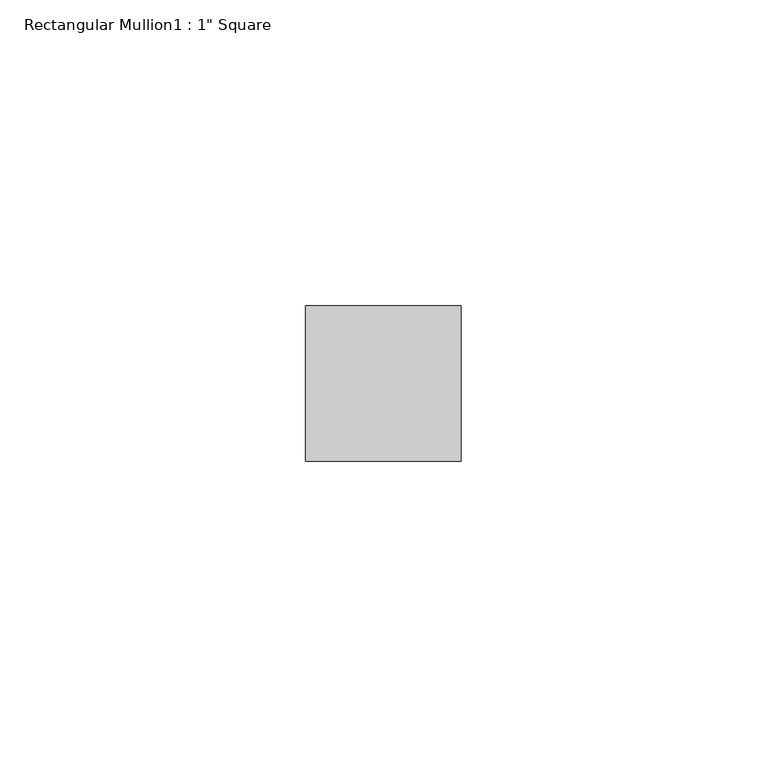
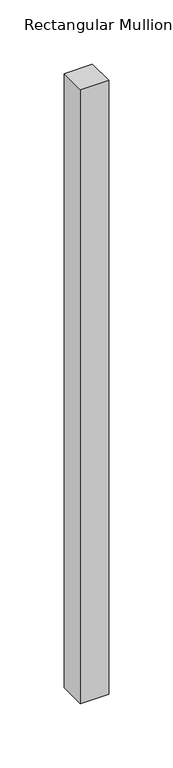
"""IFC4 building model written with IfcOpenShell, lengths in millimetres: member geometry."""

import ifcopenshell
import ifcopenshell.guid

model = None  # the IFC model being written
_history = None  # IfcOwnerHistory: only IFC2X3 demands one
_inside = {}  # id of a spatial element -> (the spatial element, [elements in it])
_under = {}  # id of a project, library or spatial element -> (it, [spatial elements below it])
_declared = {}  # id of a project -> (the project, [libraries it declares])
_typed = {}  # id of a type object -> (the type object, [elements of that type])
_made_of = {}  # id of a material, layer set ... -> (it, [elements and type objects made of it])


def new_model(schema):
    """Start an empty IFC model of exactly this schema.

    Asked for "IFC4X3", IfcOpenShell would pick the latest addendum, in which some entities
    have other attributes; the version numbers below select the first issue.
    IFC2X3 requires an IfcOwnerHistory on every rooted entity: one is made here for all.
    """
    global model, _history
    if schema == "IFC4X3":
        model = ifcopenshell.file(schema_version=(4, 3, 0, 0))
    else:
        model = ifcopenshell.file(schema=schema)
    _inside.clear()
    _under.clear()
    _declared.clear()
    _typed.clear()
    _made_of.clear()
    _history = None
    if model.schema == "IFC2X3":
        org = make("IfcOrganization", Name="unknown")
        user = make(
            "IfcPersonAndOrganization",
            ThePerson=make("IfcPerson", FamilyName="unknown"),
            TheOrganization=org,
        )
        app = make(
            "IfcApplication",
            ApplicationDeveloper=org,
            Version="unknown",
            ApplicationFullName="unknown",
            ApplicationIdentifier="unknown",
        )
        _history = make(
            "IfcOwnerHistory",
            OwningUser=user,
            OwningApplication=app,
            ChangeAction="ADDED",
            CreationDate=0,
        )
    return model


def make(cls, **values):
    """One entity of the class cls with the attributes given. An attribute that is None is left unset."""
    return model.create_entity(
        cls, **{name: value for name, value in values.items() if value is not None}
    )


def rooted(cls, **values):
    """An entity with a GlobalId (a new one), such as an element, a storey or a relation."""
    return make(cls, GlobalId=ifcopenshell.guid.new(), OwnerHistory=_history, **values)


def si_unit(unit_type, name, prefix=None):
    """IfcSIUnit, for example si_unit("LENGTHUNIT", "METRE", prefix="MILLI")."""
    return make("IfcSIUnit", UnitType=unit_type, Prefix=prefix, Name=name)


def assignment(units):
    """IfcUnitAssignment: the units of a project."""
    return None if units is None else make("IfcUnitAssignment", Units=units)


def point(xyz):
    """IfcCartesianPoint."""
    return None if xyz is None else make("IfcCartesianPoint", Coordinates=xyz)


def direction(xyz):
    """IfcDirection."""
    return None if xyz is None else make("IfcDirection", DirectionRatios=xyz)


def frame(location, z_axis=None, x_axis=None):
    """IfcAxis2Placement3D, a coordinate frame: its origin and axes. An axis left out is left unset."""
    return make(
        "IfcAxis2Placement3D",
        Location=point(location),
        Axis=direction(z_axis),
        RefDirection=direction(x_axis),
    )


def origin():
    """The frame at (0, 0, 0) with its axes left unset."""
    return frame((0.0, 0.0, 0.0))


def place(relative_to, where):
    """IfcLocalPlacement: puts the frame where relative to a parent placement (None: the world)."""
    return make(
        "IfcLocalPlacement", PlacementRelTo=relative_to, RelativePlacement=where
    )


def context(
    kind, dimensions, precision=None, world=None, true_north=None, identifier=None
):
    """IfcGeometricRepresentationContext, for example the 3D "Model" context."""
    return make(
        "IfcGeometricRepresentationContext",
        ContextIdentifier=identifier,
        ContextType=kind,
        CoordinateSpaceDimension=dimensions,
        Precision=precision,
        WorldCoordinateSystem=world,
        TrueNorth=true_north,
    )


def project(units=None, contexts=None):
    """IfcProject with its units and contexts."""
    return rooted(
        "IfcProject",
        Name="project",
        RepresentationContexts=contexts,
        UnitsInContext=assignment(units),
    )


def spatial(cls, under=None, at=None, **own):
    """A site, building, storey or space (cls), placed at a placement, below another one or the project."""
    s = rooted(cls, ObjectPlacement=at, **own)
    if under is not None:
        _under.setdefault(under.id(), (under, []))[1].append(s)
    return s


def polyline(points):
    """IfcPolyline through the points."""
    return make("IfcPolyline", Points=[point(p) for p in points])


def outline(outer, holes=None, kind="AREA"):
    """IfcArbitraryClosedProfileDef: a profile drawn as a closed curve; with holes, ...WithVoids."""
    if holes is None:
        return make("IfcArbitraryClosedProfileDef", ProfileType=kind, OuterCurve=outer)
    return make(
        "IfcArbitraryProfileDefWithVoids",
        ProfileType=kind,
        OuterCurve=outer,
        InnerCurves=holes,
    )


def extrude(swept, where, along, depth):
    """IfcExtrudedAreaSolid: the profile swept, set in the frame where, extruded along a direction by depth."""
    return make(
        "IfcExtrudedAreaSolid",
        SweptArea=swept,
        Position=where,
        ExtrudedDirection=direction(along),
        Depth=depth,
    )


def shape(context_of_items, identifier, shape_type, items):
    """IfcShapeRepresentation: the items that make up one representation, for example the "Body"."""
    return make(
        "IfcShapeRepresentation",
        ContextOfItems=context_of_items,
        RepresentationIdentifier=identifier,
        RepresentationType=shape_type,
        Items=items,
    )


def source(mapping_origin, context_of_items, identifier, shape_type, items):
    """IfcRepresentationMap: a shape defined once, which mapped items show again and again."""
    return make(
        "IfcRepresentationMap",
        MappingOrigin=mapping_origin,
        MappedRepresentation=shape(context_of_items, identifier, shape_type, items),
    )


def transform(
    local_origin,
    x_axis=None,
    y_axis=None,
    z_axis=None,
    scale=None,
    scale2=None,
    scale3=None,
    uniform=True,
):
    """IfcCartesianTransformationOperator3D, or its non-uniform kind. x_axis, y_axis, z_axis: its Axis1, 2, 3."""
    if uniform:
        return make(
            "IfcCartesianTransformationOperator3D",
            Axis1=direction(x_axis),
            Axis2=direction(y_axis),
            LocalOrigin=point(local_origin),
            Scale=scale,
            Axis3=direction(z_axis),
        )
    return make(
        "IfcCartesianTransformationOperator3DnonUniform",
        Axis1=direction(x_axis),
        Axis2=direction(y_axis),
        LocalOrigin=point(local_origin),
        Scale=scale,
        Axis3=direction(z_axis),
        Scale2=scale2,
        Scale3=scale3,
    )


def mapped(mapping_source, mapping_target):
    """IfcMappedItem: shows the shape of a source again, moved by a transform."""
    return make(
        "IfcMappedItem", MappingSource=mapping_source, MappingTarget=mapping_target
    )


def made_of(thing, what):
    """Note that an element or type object is made of a material, layer set ...; save() writes the relation."""
    if what is not None:
        _made_of.setdefault(what.id(), (what, []))[1].append(thing)
    return thing


def element(
    cls,
    number,
    at=None,
    inside=None,
    cuts=None,
    type_object=None,
    material=None,
    context=None,
    identifier="Body",
    shape_type=None,
    held_by="IfcProductDefinitionShape",
    body=None,
    shapes=None,
    **own,
):
    """One element of the class cls, such as IfcWall. Its Tag is "e" and its number.

    at: its placement. inside: the storey or other place that contains it. cuts: it is an
    opening in that element (IfcRelVoidsElement). A single representation is given by context,
    identifier, shape_type and body (its items); several are given by shapes. held_by: the class
    of the entity that holds the representations. save() writes the other relations.
    """
    e = rooted(cls, Tag="e%d" % number, ObjectPlacement=at, **own)
    if body is not None:
        shapes = [shape(context, identifier, shape_type, body)]
    if shapes is not None:
        e.Representation = make(held_by, Representations=shapes)
    if inside is not None:
        _inside.setdefault(inside.id(), (inside, []))[1].append(e)
    if cuts is not None:
        rooted(
            "IfcRelVoidsElement", RelatingBuildingElement=cuts, RelatedOpeningElement=e
        )
    if type_object is not None:
        _typed.setdefault(type_object.id(), (type_object, []))[1].append(e)
    return made_of(e, material)


def aggregate(whole, parts):
    """IfcRelAggregates: a whole, such as a stair, and the parts it consists of."""
    return rooted("IfcRelAggregates", RelatingObject=whole, RelatedObjects=parts)


def save(model, path):
    """Write the relations noted so far, then the file.

    IfcRelAggregates (storeys below a building ...), IfcRelContainedInSpatialStructure (elements
    in a storey), IfcRelDefinesByType, IfcRelAssociatesMaterial and IfcRelDeclares: one each for
    every whole, place, type object, material and project.
    """
    for whole, parts in _under.values():
        aggregate(whole, parts)
    for where, things in _inside.values():
        rooted(
            "IfcRelContainedInSpatialStructure",
            RelatedElements=things,
            RelatingStructure=where,
        )
    for kind, things in _typed.values():
        rooted("IfcRelDefinesByType", RelatedObjects=things, RelatingType=kind)
    for what, things in _made_of.values():
        rooted("IfcRelAssociatesMaterial", RelatedObjects=things, RelatingMaterial=what)
    for by, libraries in _declared.values():
        rooted("IfcRelDeclares", RelatingContext=by, RelatedDefinitions=libraries)
    model.write(path)


def member_8963dcaa(model_context):
    return source(origin(), model_context, "Body", "SweptSolid", [
        extrude(outline(polyline([(0.0, -19.05), (0.0, -44.45), (-25.4, -44.45), (-25.4, -19.05), (0.0, -19.05)])), frame((0.0, 0.0, -584.2), z_axis=(0.0, 0.0, 1.0), x_axis=(1.0, 0.0, 0.0)), (0.0, 0.0, 1.0), 584.2),
    ])


if __name__ == "__main__":
    model = new_model("IFC4")
    model_context = context("Model", 3, world=origin())
    ifc_project = project(units=[si_unit("LENGTHUNIT", "METRE", prefix="MILLI")], contexts=[model_context])
    site = spatial("IfcSite", under=ifc_project)
    building = spatial("IfcBuilding", under=site)
    placement = place(None, origin())
    member_shape = member_8963dcaa(model_context)
    element("IfcMember", 1, ObjectType="Rectangular Mullion1 : 1\" Square", at=placement, inside=building, context=model_context, shape_type="MappedRepresentation", body=[
        mapped(member_shape, transform((0.0, 0.0, 0.0), x_axis=(1.0, 0.0, 0.0), y_axis=(0.0, 1.0, 0.0), z_axis=(0.0, 0.0, 1.0))),
    ])
    save(model, "model.ifc")

# Revit data of these elements
# Type "Rectangular Mullion1 : 1\" Square"
#   built-in parameter 1007351 = 0.104167 (stored number, unit not read)
#   built-in parameter 1007304 = 0.0833333 (stored number, unit not read)
#   built-in parameter 1007301 = 0.0416667 (stored number, unit not read)
#   built-in parameter 1007300 = 0.0416667 (stored number, unit not read)
